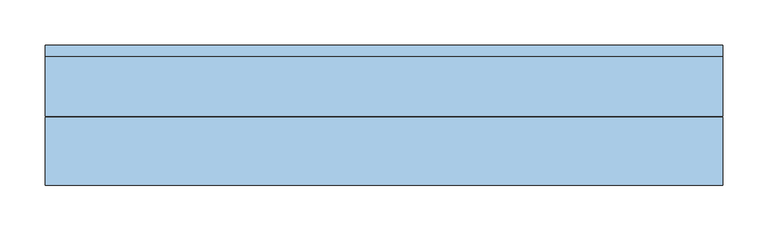
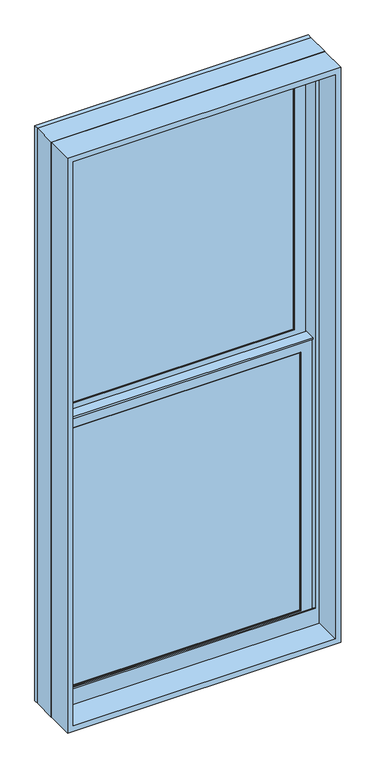
"""IFC4 building model written with IfcOpenShell, lengths in millimetres: window geometry, Window-Double_Hung-Marvin-Essential : ESDH2656."""

from ifc_helpers import new_model, si_unit, frame, origin, place, context, project, spatial, polyline, outline, extrude, faceted_brep, source, transform, mapped, element, save


def window_64265f39(model_context):
    return source(origin(), model_context, "Body", "SolidModel", [
        extrude(outline(polyline([(115.3583333, 20.6375), (115.3583333, 15.875), (96.3083333, 15.875), (96.3083333, 20.6375), (115.3583333, 20.6375)])), frame((0.0, 0.0, 831.85), z_axis=(0.0, 0.0, 1.0), x_axis=(1.0, 0.0, 0.0)), (0.0, 0.0, 1.0), 755.65),
        extrude(outline(polyline([(-96.3083333, 20.6375), (-96.3083333, 15.875), (-115.3583333, 15.875), (-115.3583333, 20.6375), (-96.3083333, 20.6375)])), frame((0.0, 0.0, 831.85), z_axis=(0.0, 0.0, 1.0), x_axis=(1.0, 0.0, 0.0)), (0.0, 0.0, 1.0), 755.65),
        extrude(outline(polyline([(317.5, 20.6375), (317.5, 15.875), (-317.5, 15.875), (-317.5, 20.6375), (317.5, 20.6375)])), frame((0.0, 0.0, 1200.15), z_axis=(0.0, 0.0, 1.0), x_axis=(1.0, 0.0, 0.0)), (0.0, 0.0, 1.0), 19.05),
        extrude(outline(polyline([(-115.3583333, 46.83125), (-115.3583333, 51.59375), (-96.3083333, 51.59375), (-96.3083333, 46.83125), (-115.3583333, 46.83125)])), frame((0.0, 0.0, 1625.6), z_axis=(0.0, 0.0, 1.0), x_axis=(1.0, 0.0, 0.0)), (0.0, 0.0, 1.0), 755.65),
        extrude(outline(polyline([(96.3083333, 46.83125), (96.3083333, 51.59375), (115.3583333, 51.59375), (115.3583333, 46.83125), (96.3083333, 46.83125)])), frame((0.0, 0.0, 1625.6), z_axis=(0.0, 0.0, 1.0), x_axis=(1.0, 0.0, 0.0)), (0.0, 0.0, 1.0), 755.65),
        extrude(outline(polyline([(-317.5, 46.83125), (-317.5, 51.59375), (317.5, 51.59375), (317.5, 46.83125), (-317.5, 46.83125)])), frame((0.0, 0.0, 1993.9), z_axis=(0.0, 0.0, 1.0), x_axis=(1.0, 0.0, 0.0)), (0.0, 0.0, 1.0), 19.05),
        extrude(outline(polyline([(115.3583333, 20.6375), (96.3083333, 20.6375), (96.3083333, 25.4), (115.3583333, 25.4), (115.3583333, 20.6375)])), frame((0.0, 0.0, 831.85), z_axis=(0.0, 0.0, 1.0), x_axis=(1.0, 0.0, 0.0)), (0.0, 0.0, 1.0), 755.65),
        extrude(outline(polyline([(-96.3083333, 20.6375), (-115.3583333, 20.6375), (-115.3583333, 25.4), (-96.3083333, 25.4), (-96.3083333, 20.6375)])), frame((0.0, 0.0, 831.85), z_axis=(0.0, 0.0, 1.0), x_axis=(1.0, 0.0, 0.0)), (0.0, 0.0, 1.0), 755.65),
        extrude(outline(polyline([(317.5, 20.6375), (-317.5, 20.6375), (-317.5, 25.4), (317.5, 25.4), (317.5, 20.6375)])), frame((0.0, 0.0, 1200.15), z_axis=(0.0, 0.0, 1.0), x_axis=(1.0, 0.0, 0.0)), (0.0, 0.0, 1.0), 19.05),
        extrude(outline(polyline([(-115.3583333, 56.35625), (-96.3083333, 56.35625), (-96.3083333, 51.59375), (-115.3583333, 51.59375), (-115.3583333, 56.35625)])), frame((0.0, 0.0, 1625.6), z_axis=(0.0, 0.0, 1.0), x_axis=(1.0, 0.0, 0.0)), (0.0, 0.0, 1.0), 755.65),
        extrude(outline(polyline([(96.3083333, 56.35625), (115.3583333, 56.35625), (115.3583333, 51.59375), (96.3083333, 51.59375), (96.3083333, 56.35625)])), frame((0.0, 0.0, 1625.6), z_axis=(0.0, 0.0, 1.0), x_axis=(1.0, 0.0, 0.0)), (0.0, 0.0, 1.0), 755.65),
        extrude(outline(polyline([(-317.5, 56.35625), (317.5, 56.35625), (317.5, 51.59375), (-317.5, 51.59375), (-317.5, 56.35625)])), frame((0.0, 0.0, 1993.9), z_axis=(0.0, 0.0, 1.0), x_axis=(1.0, 0.0, 0.0)), (0.0, 0.0, 1.0), 19.05),
        faceted_brep([(-344.4875, 5.6780605, 1617.5351748), (-344.4875, 5.6780605, 1612.9), (344.4875, 5.6780605, 1612.9), (344.4875, 5.6780605, 1617.5351748), (-344.4875, 34.8118605, 1617.5351748), (344.4875, 34.8118605, 1617.5351748), (344.4875, 34.8118605, 1612.9), (-344.4875, 34.8118605, 1612.9), (-344.4875, 30.1625, 1612.9), (-344.4875, 30.1625, 804.8625), (-344.4875, 8.9241104, 804.8625), (-344.4875, 8.9241104, 1612.9), (344.4875, 8.9241104, 1612.9), (344.4875, 30.1625, 1612.9), (344.4875, 8.9241104, 804.8625), (344.4875, 30.1625, 804.8625), (-328.6034752, 11.90625, 1598.6034752), (-328.6034752, 30.1625, 1598.6034752), (328.6034752, 30.1625, 1598.6034752), (328.6034752, 11.90625, 1598.6034752), (-311.94375, 10.4662439, 1581.94375), (-311.94375, 11.90625, 1581.94375), (311.94375, 11.90625, 1581.94375), (311.94375, 10.4662439, 1581.94375), (313.4858834, 8.9241104, 1583.4858834), (-313.4858834, 8.9241104, 1583.4858834), (328.6034752, 30.1625, 820.7465248), (328.6034752, 11.90625, 820.7465248), (311.94375, 11.90625, 837.40625), (311.94375, 10.4662439, 837.40625), (313.4858834, 8.9241104, 835.8641166), (-328.6034752, 30.1625, 820.7465248), (-328.6034752, 11.90625, 820.7465248), (-311.94375, 11.90625, 837.40625), (-311.94375, 10.4662439, 837.40625), (-313.4858834, 8.9241104, 835.8641166)], [[[0, 1, 2, 3]], [[4, 5, 6, 7]], [[1, 0, 4, 7, 8, 9, 10, 11]], [[2, 1, 11, 12]], [[7, 6, 13, 8]], [[3, 2, 12, 14, 15, 13, 6, 5]], [[0, 3, 5, 4]], [[16, 17, 18, 19]], [[20, 21, 22, 23]], [[20, 23, 24, 25]], [[19, 18, 26, 27]], [[23, 22, 28, 29]], [[24, 23, 29, 30]], [[27, 26, 31, 32]], [[29, 28, 33, 34]], [[30, 29, 34, 35]], [[15, 14, 10, 9]], [[15, 9, 8, 13], [18, 17, 31, 26]], [[17, 16, 32, 31]], [[16, 19, 27, 32], [22, 21, 33, 28]], [[21, 20, 34, 33]], [[20, 25, 35, 34]], [[10, 14, 12, 11], [25, 24, 30, 35]]]),
        extrude(outline(polyline([(38.5955581, 1598.6125), (33.5778968, 1598.6125), (33.5778968, 1600.2), (39.9405976, 1600.2), (39.9405976, 1598.6125), (61.515625, 1598.6125), (47.6307501, 1595.2975159), (38.5955581, 1595.2975159), (38.5955581, 1598.6125)])), frame((-344.4875, 0.0, 0.0), z_axis=(1.0, 0.0, 0.0), x_axis=(0.0, 1.0, 0.0)), (0.0, 0.0, 1.0), 688.975),
        faceted_brep([(374.65, 0.0, 774.7), (374.65, 0.0, 2438.4), (-374.65, 0.0, 2438.4), (-374.65, 0.0, 774.7), (348.45625, 0.0, 835.81875), (-348.45625, 0.0, 835.81875), (-348.45625, 0.0, 2412.20625), (348.45625, 0.0, 2412.20625), (348.45625, 3.96875, 774.7), (-348.45625, 3.96875, 774.7), (-348.45625, 3.96875, 835.81875), (348.45625, 3.96875, 835.81875), (-374.65, 65.6828125, 774.7), (-348.45625, 65.6828125, 774.7), (348.45625, 65.6828125, 774.7), (374.65, 65.6828125, 774.7), (-374.65, 65.6828125, 2438.4), (374.65, 65.6828125, 2438.4), (348.45625, 65.6828125, 2412.20625), (-348.45625, 65.6828125, 2412.20625)], [[[0, 1, 2, 3], [4, 5, 6, 7]], [[8, 9, 10, 11]], [[5, 4, 11, 10]], [[0, 3, 12, 13, 9, 8, 14, 15]], [[13, 12, 16, 17, 15, 14, 18, 19]], [[13, 19, 6, 5, 10, 9]], [[7, 6, 19, 18]], [[18, 14, 8, 11, 4, 7]], [[1, 0, 15, 17]], [[2, 1, 17, 16]], [[3, 2, 16, 12]]]),
        faceted_brep([(348.45625, 30.1625, 1606.55), (346.86875, 30.1625, 1606.55), (346.86875, 30.1625, 799.0544613), (348.45625, 30.1625, 799.0544613), (-346.86875, 30.1625, 1606.55), (-348.45625, 30.1625, 1606.55), (-348.45625, 30.1625, 799.0544613), (-346.86875, 30.1625, 799.0544613), (346.86875, 63.5, 1606.55), (348.45625, 63.5, 1606.55), (348.45625, 63.5, 792.5743077), (346.86875, 63.5, 792.5743077), (-348.45625, 63.5, 1606.55), (-346.86875, 63.5, 1606.55), (-346.86875, 63.5, 792.5743077), (-348.45625, 63.5, 792.5743077), (359.7108932, 3.96875, 804.1460105), (359.7108932, 3.96875, 774.7), (359.7108932, 65.6828125, 774.7), (359.7108932, 65.6828125, 792.150012), (-359.7108932, 3.96875, 774.7), (-359.7108932, 3.96875, 804.1460105), (-359.7108932, 65.6828125, 792.150012), (-359.7108932, 65.6828125, 774.7), (359.7108932, 78.58125, 789.6428097), (-359.7108932, 78.58125, 789.6428097), (-357.6971252, 68.2348864, 791.6539391), (-339.73135, 68.2348864, 791.6539391), (-339.73135, 65.6828125, 792.150012), (339.73135, 65.6828125, 792.150012), (339.73135, 68.2348864, 791.6539391), (357.6971252, 68.2348864, 791.6539391), (-374.65, 65.6828125, 774.7), (-374.65, 78.5948249, 774.7), (374.65, 78.5948249, 774.7), (374.65, 65.6828125, 774.7), (-374.65, 78.58125, 2438.4), (374.65, 78.58125, 2438.4), (359.7108932, 78.58125, 2423.4608932), (-359.7108932, 78.58125, 2423.4608932), (-374.65, 65.6828125, 2438.4), (-357.6971252, 68.2348864, 2421.4471252), (357.6971252, 68.2348864, 2421.4471252), (339.73135, 68.2348864, 2403.48135), (-339.73135, 68.2348864, 2403.48135), (-339.73135, 65.6828125, 2403.48135), (339.73135, 65.6828125, 2403.48135), (374.65, 65.6828125, 2438.4)], [[[0, 1, 2, 3]], [[4, 5, 6, 7]], [[8, 9, 10, 11]], [[12, 13, 14, 15]], [[1, 8, 11, 2]], [[9, 0, 3, 10]], [[1, 0, 9, 8]], [[5, 4, 13, 12]], [[5, 12, 15, 6]], [[13, 4, 7, 14]], [[16, 17, 18, 19]], [[20, 21, 22, 23]], [[24, 25, 26, 27, 28, 22, 21, 16, 19, 29, 30, 31], [3, 2, 11, 10], [7, 6, 15, 14]], [[17, 16, 21, 20]], [[17, 20, 23, 32, 33, 34, 35, 18]], [[34, 33, 36, 37], [25, 24, 38, 39]], [[33, 32, 40, 36]], [[39, 41, 26, 25]], [[41, 42, 31, 30, 43, 44, 27, 26]], [[44, 45, 28, 27]], [[40, 32, 23, 22, 28, 45, 46, 29, 19, 18, 35, 47]], [[36, 40, 47, 37]], [[39, 38, 42, 41]], [[44, 43, 46, 45]], [[34, 37, 47, 35]], [[42, 38, 24, 31]], [[46, 43, 30, 29]]]),
        extrude(outline(polyline([(324.64375, 11.90625), (-324.64375, 11.90625), (-324.64375, 15.08125), (324.64375, 15.08125), (324.64375, 11.90625)])), frame((0.0, 0.0, 824.70625), z_axis=(0.0, 0.0, 1.0), x_axis=(1.0, 0.0, 0.0)), (0.0, 0.0, 1.0), 769.9375),
        extrude(outline(polyline([(324.64375, 42.8625), (-324.64375, 42.8625), (-324.64375, 46.0375), (324.64375, 46.0375), (324.64375, 42.8625)])), frame((0.0, 0.0, 1618.45625), z_axis=(0.0, 0.0, 1.0), x_axis=(1.0, 0.0, 0.0)), (0.0, 0.0, 1.0), 769.9375),
        faceted_brep([(-311.94375, 31.194477, 1581.94375), (-313.4858834, 32.7366104, 1583.4858834), (313.4858834, 32.7366104, 1583.4858834), (311.94375, 31.194477, 1581.94375), (-311.94375, 30.1625, 1581.94375), (311.94375, 30.1625, 1581.94375), (-344.4875, 32.7366104, 1614.4875), (-344.4875, 30.1625, 1614.4875), (344.4875, 30.1625, 1614.4875), (344.4875, 32.7366104, 1614.4875), (313.4858834, 32.7366104, 835.8641166), (311.94375, 31.194477, 837.40625), (311.94375, 30.1625, 837.40625), (344.4875, 30.1625, 804.8625), (344.4875, 32.7366104, 804.8625), (-313.4858834, 32.7366104, 835.8641166), (-311.94375, 31.194477, 837.40625), (-311.94375, 30.1625, 837.40625), (-344.4875, 30.1625, 804.8625), (-344.4875, 32.7366104, 804.8625)], [[[0, 1, 2, 3]], [[4, 0, 3, 5]], [[6, 7, 8, 9]], [[3, 2, 10, 11]], [[5, 3, 11, 12]], [[9, 8, 13, 14]], [[11, 10, 15, 16]], [[12, 11, 16, 17]], [[14, 13, 18, 19]], [[9, 14, 19, 6], [1, 15, 10, 2]], [[16, 15, 1, 0]], [[17, 16, 0, 4]], [[7, 18, 13, 8], [5, 12, 17, 4]], [[19, 18, 7, 6]]]),
        faceted_brep([(-328.6034752, 42.8625, 2392.3534752), (-328.6034752, 61.11875, 2392.3534752), (328.6034752, 61.11875, 2392.3534752), (328.6034752, 42.8625, 2392.3534752), (-311.94375, 41.4224939, 2375.69375), (-311.94375, 42.8625, 2375.69375), (311.94375, 42.8625, 2375.69375), (311.94375, 41.4224939, 2375.69375), (-313.4858834, 39.8803604, 2377.2358834), (313.4858834, 39.8803604, 2377.2358834), (-344.4875, 61.11875, 2408.2375), (-344.4875, 39.8803604, 2408.2375), (344.4875, 39.8803604, 2408.2375), (344.4875, 61.11875, 2408.2375), (328.6034752, 61.11875, 1614.4965248), (328.6034752, 42.8625, 1614.4965248), (311.94375, 42.8625, 1631.15625), (311.94375, 41.4224939, 1631.15625), (313.4858834, 39.8803604, 1629.6141166), (344.4875, 39.8803604, 1598.6125), (344.4875, 61.11875, 1598.6125), (-328.6034752, 61.11875, 1614.4965248), (-328.6034752, 42.8625, 1614.4965248), (-311.94375, 42.8625, 1631.15625), (-311.94375, 41.4224939, 1631.15625), (-313.4858834, 39.8803604, 1629.6141166), (-344.4875, 39.8803604, 1598.6125), (-344.4875, 61.11875, 1598.6125)], [[[0, 1, 2, 3]], [[4, 5, 6, 7]], [[8, 4, 7, 9]], [[10, 11, 12, 13]], [[3, 2, 14, 15]], [[7, 6, 16, 17]], [[9, 7, 17, 18]], [[13, 12, 19, 20]], [[15, 14, 21, 22]], [[17, 16, 23, 24]], [[18, 17, 24, 25]], [[20, 19, 26, 27]], [[13, 20, 27, 10], [1, 21, 14, 2]], [[22, 21, 1, 0]], [[3, 15, 22, 0], [5, 23, 16, 6]], [[24, 23, 5, 4]], [[25, 24, 4, 8]], [[11, 26, 19, 12], [9, 18, 25, 8]], [[27, 26, 11, 10]]]),
        faceted_brep([(-344.4875, 61.11875, 1598.6125), (-344.4875, 63.6928604, 1598.6125), (344.4875, 63.6928604, 1598.6125), (344.4875, 61.11875, 1598.6125), (-311.94375, 62.150727, 1631.15625), (-311.94375, 61.11875, 1631.15625), (311.94375, 61.11875, 1631.15625), (311.94375, 62.150727, 1631.15625), (-313.4858834, 63.6928604, 1629.6141166), (313.4858834, 63.6928604, 1629.6141166), (344.4875, 63.6928604, 2408.2375), (344.4875, 61.11875, 2408.2375), (311.94375, 61.11875, 2375.69375), (311.94375, 62.150727, 2375.69375), (313.4858834, 63.6928604, 2377.2358834), (-344.4875, 63.6928604, 2408.2375), (-344.4875, 61.11875, 2408.2375), (-311.94375, 61.11875, 2375.69375), (-311.94375, 62.150727, 2375.69375), (-313.4858834, 63.6928604, 2377.2358834)], [[[0, 1, 2, 3]], [[4, 5, 6, 7]], [[8, 4, 7, 9]], [[3, 2, 10, 11]], [[7, 6, 12, 13]], [[9, 7, 13, 14]], [[11, 10, 15, 16]], [[13, 12, 17, 18]], [[14, 13, 18, 19]], [[16, 15, 1, 0]], [[3, 11, 16, 0], [5, 17, 12, 6]], [[18, 17, 5, 4]], [[19, 18, 4, 8]], [[1, 15, 10, 2], [9, 14, 19, 8]]]),
        extrude(outline(polyline([(324.64375, 26.19375), (-324.64375, 26.19375), (-324.64375, 30.1625), (324.64375, 30.1625), (324.64375, 26.19375)])), frame((0.0, 0.0, 824.70625), z_axis=(0.0, 0.0, 1.0), x_axis=(1.0, 0.0, 0.0)), (0.0, 0.0, 1.0), 769.9375),
        extrude(outline(polyline([(324.64375, 57.15), (-324.64375, 57.15), (-324.64375, 61.11875), (324.64375, 61.11875), (324.64375, 57.15)])), frame((0.0, 0.0, 1618.45625), z_axis=(0.0, 0.0, 1.0), x_axis=(1.0, 0.0, 0.0)), (0.0, 0.0, 1.0), 769.9375),
        extrude(outline(polyline([(2438.4, 374.65), (2438.4, -374.65), (774.7, -374.65), (774.7, 374.65), (2438.4, 374.65)]), holes=[polyline([(2422.525, 358.775), (790.575, 358.775), (790.575, -358.775), (2422.525, -358.775), (2422.525, 358.775)])]), frame((0.0, -76.2, 0.0), z_axis=(0.0, 1.0, 0.0), x_axis=(0.0, 0.0, 1.0)), (0.0, 0.0, 1.0), 75.40625),
    ])


if __name__ == "__main__":
    model = new_model("IFC4")
    model_context = context("Model", 3, world=origin())
    ifc_project = project(units=[si_unit("LENGTHUNIT", "METRE", prefix="MILLI")], contexts=[model_context])
    site = spatial("IfcSite", under=ifc_project)
    building = spatial("IfcBuilding", under=site)
    placement = place(None, origin())
    window_shape = window_64265f39(model_context)
    element("IfcWindow", 1, ObjectType="Window-Double_Hung-Marvin-Essential : ESDH2656", at=placement, inside=building, context=model_context, shape_type="MappedRepresentation", body=[
        mapped(window_shape, transform((0.0, 0.0, 0.0), x_axis=(1.0, 0.0, 0.0), y_axis=(0.0, 1.0, 0.0), z_axis=(0.0, 0.0, 1.0))),
    ])
    save(model, "model.ifc")

# Revit data of these elements
# Type "Window-Double_Hung-Marvin-Essential : ESDH2656"
#   Type Mark = "70"
#   Window Type = "Essential Double Hung"
#   Product data url = "https://bimobject.com/marvin-windows-and-doors/product/marvin-dhwau"
#   Product Guid = "c4a96547-874c-4385-91dc-a058adc19d98"
#   Frame = "All Ultrex"
#   Egress Window = "No"
#   URL = "www.marvin.com"
#   Model = "ESDH2656"
#   Manufacturer = "Marvin Windows and Doors"
#   Label Egress = ""
#   Glass Type = "IG Low E II with Argon"
#   Design Pressure = "DP40"
#   Description = "3066 DBHG"
#   Analytic Construction = "<None>"
#   Prairie Corner Width = 0' - 4"
#   Prairie Corner Height = 0' - 4"
#   Egress Width = 2' - 2 9/16"
#   Egress Height = 2' - 4 27/128"
#   Rough Width = 2' - 6"
#   Rough Height = 5' - 6"
#   Nominal Width = 2' - 6"
#   Nominal Height = 5' - 6"
#   Inset to Installation Flange [instance default] = 0' - 1"
#   Height = 5' - 5 1/2"
#   Egress Area = 5.20384 SF
#   Default Head Height = 8' - 0"
#   Width = 2' - 5 1/2"
#   Daylight Area = 9.99984 SF
#   DLO Width = 2' - 0 9/16"
#   DLO Height = 2' - 5 5/16"
#   Muntins Top Sash = yes
#   Lites Wide Top Sash = 3
#   Lites Wide Bottom Sash = 3
#   Lites High Top Sash = 2
#   Lites High Bottom Sash = 2
#   Lite Cut Prairie 9 = no
#   Lite Cut HV Grid = yes
#   Muntins Bottom Sash = yes
#   Label Visibility = no
#   Jamb Extension Visibility = yes
#   Edition number = 1
#   Interior Material = Ultrex-Marvin-Stonewhite
#   Glazing Material = Glass-Marvin-IG Low E II with Argon
#   Cladding Material = Ultrex-Marvin-Pebblegray
#   Wall Closure = (empty or 0)
#   Assembly Code = ""
# Element 1 (IfcWindow, "Window-Double_Hung-Marvin-Essential : ESDH2656")
#   Materials on its faces: "Ultrex-Marvin-Pebblegray", "Ultrex-Marvin-Stonewhite", "Glass-Marvin-IG Low E II with Argon"
# Materials
#   "Ultrex-Marvin-Stonewhite": class "Paint", colour RGB 250 251 245, transparency 0
#   "Glass-Marvin-IG Low E II with Argon": class "Glass", colour RGB 0 128 192, transparency 0.85
#   "Ultrex-Marvin-Pebblegray": class "Paint", colour RGB 189 185 173, transparency 0
